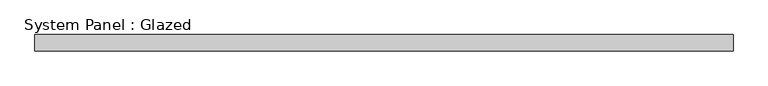
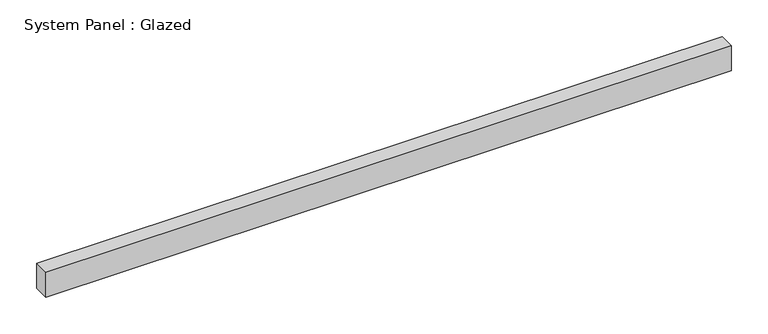
"""IFC4 building model written with IfcOpenShell, lengths in millimetres: plate geometry, System Panel : Glazed."""

import ifcopenshell
import ifcopenshell.guid

model = None  # the IFC model being written
_history = None  # IfcOwnerHistory: only IFC2X3 demands one
_inside = {}  # id of a spatial element -> (the spatial element, [elements in it])
_under = {}  # id of a project, library or spatial element -> (it, [spatial elements below it])
_declared = {}  # id of a project -> (the project, [libraries it declares])
_typed = {}  # id of a type object -> (the type object, [elements of that type])
_made_of = {}  # id of a material, layer set ... -> (it, [elements and type objects made of it])


def new_model(schema):
    """Start an empty IFC model of exactly this schema.

    Asked for "IFC4X3", IfcOpenShell would pick the latest addendum, in which some entities
    have other attributes; the version numbers below select the first issue.
    IFC2X3 requires an IfcOwnerHistory on every rooted entity: one is made here for all.
    """
    global model, _history
    if schema == "IFC4X3":
        model = ifcopenshell.file(schema_version=(4, 3, 0, 0))
    else:
        model = ifcopenshell.file(schema=schema)
    _inside.clear()
    _under.clear()
    _declared.clear()
    _typed.clear()
    _made_of.clear()
    _history = None
    if model.schema == "IFC2X3":
        org = make("IfcOrganization", Name="unknown")
        user = make(
            "IfcPersonAndOrganization",
            ThePerson=make("IfcPerson", FamilyName="unknown"),
            TheOrganization=org,
        )
        app = make(
            "IfcApplication",
            ApplicationDeveloper=org,
            Version="unknown",
            ApplicationFullName="unknown",
            ApplicationIdentifier="unknown",
        )
        _history = make(
            "IfcOwnerHistory",
            OwningUser=user,
            OwningApplication=app,
            ChangeAction="ADDED",
            CreationDate=0,
        )
    return model


def make(cls, **values):
    """One entity of the class cls with the attributes given. An attribute that is None is left unset."""
    return model.create_entity(
        cls, **{name: value for name, value in values.items() if value is not None}
    )


def rooted(cls, **values):
    """An entity with a GlobalId (a new one), such as an element, a storey or a relation."""
    return make(cls, GlobalId=ifcopenshell.guid.new(), OwnerHistory=_history, **values)


def si_unit(unit_type, name, prefix=None):
    """IfcSIUnit, for example si_unit("LENGTHUNIT", "METRE", prefix="MILLI")."""
    return make("IfcSIUnit", UnitType=unit_type, Prefix=prefix, Name=name)


def assignment(units):
    """IfcUnitAssignment: the units of a project."""
    return None if units is None else make("IfcUnitAssignment", Units=units)


def point(xyz):
    """IfcCartesianPoint."""
    return None if xyz is None else make("IfcCartesianPoint", Coordinates=xyz)


def direction(xyz):
    """IfcDirection."""
    return None if xyz is None else make("IfcDirection", DirectionRatios=xyz)


def frame(location, z_axis=None, x_axis=None):
    """IfcAxis2Placement3D, a coordinate frame: its origin and axes. An axis left out is left unset."""
    return make(
        "IfcAxis2Placement3D",
        Location=point(location),
        Axis=direction(z_axis),
        RefDirection=direction(x_axis),
    )


def origin():
    """The frame at (0, 0, 0) with its axes left unset."""
    return frame((0.0, 0.0, 0.0))


def origin_with_axes():
    """The frame at (0, 0, 0) with the z axis (0, 0, 1) and the x axis (1, 0, 0) written out."""
    return frame((0.0, 0.0, 0.0), z_axis=(0.0, 0.0, 1.0), x_axis=(1.0, 0.0, 0.0))


def place(relative_to, where):
    """IfcLocalPlacement: puts the frame where relative to a parent placement (None: the world)."""
    return make(
        "IfcLocalPlacement", PlacementRelTo=relative_to, RelativePlacement=where
    )


def context(
    kind, dimensions, precision=None, world=None, true_north=None, identifier=None
):
    """IfcGeometricRepresentationContext, for example the 3D "Model" context."""
    return make(
        "IfcGeometricRepresentationContext",
        ContextIdentifier=identifier,
        ContextType=kind,
        CoordinateSpaceDimension=dimensions,
        Precision=precision,
        WorldCoordinateSystem=world,
        TrueNorth=true_north,
    )


def project(units=None, contexts=None):
    """IfcProject with its units and contexts."""
    return rooted(
        "IfcProject",
        Name="project",
        RepresentationContexts=contexts,
        UnitsInContext=assignment(units),
    )


def spatial(cls, under=None, at=None, **own):
    """A site, building, storey or space (cls), placed at a placement, below another one or the project."""
    s = rooted(cls, ObjectPlacement=at, **own)
    if under is not None:
        _under.setdefault(under.id(), (under, []))[1].append(s)
    return s


def polyline(points):
    """IfcPolyline through the points."""
    return make("IfcPolyline", Points=[point(p) for p in points])


def outline(outer, holes=None, kind="AREA"):
    """IfcArbitraryClosedProfileDef: a profile drawn as a closed curve; with holes, ...WithVoids."""
    if holes is None:
        return make("IfcArbitraryClosedProfileDef", ProfileType=kind, OuterCurve=outer)
    return make(
        "IfcArbitraryProfileDefWithVoids",
        ProfileType=kind,
        OuterCurve=outer,
        InnerCurves=holes,
    )


def extrude(swept, where, along, depth):
    """IfcExtrudedAreaSolid: the profile swept, set in the frame where, extruded along a direction by depth."""
    return make(
        "IfcExtrudedAreaSolid",
        SweptArea=swept,
        Position=where,
        ExtrudedDirection=direction(along),
        Depth=depth,
    )


def shape(context_of_items, identifier, shape_type, items):
    """IfcShapeRepresentation: the items that make up one representation, for example the "Body"."""
    return make(
        "IfcShapeRepresentation",
        ContextOfItems=context_of_items,
        RepresentationIdentifier=identifier,
        RepresentationType=shape_type,
        Items=items,
    )


def source(mapping_origin, context_of_items, identifier, shape_type, items):
    """IfcRepresentationMap: a shape defined once, which mapped items show again and again."""
    return make(
        "IfcRepresentationMap",
        MappingOrigin=mapping_origin,
        MappedRepresentation=shape(context_of_items, identifier, shape_type, items),
    )


def transform(
    local_origin,
    x_axis=None,
    y_axis=None,
    z_axis=None,
    scale=None,
    scale2=None,
    scale3=None,
    uniform=True,
):
    """IfcCartesianTransformationOperator3D, or its non-uniform kind. x_axis, y_axis, z_axis: its Axis1, 2, 3."""
    if uniform:
        return make(
            "IfcCartesianTransformationOperator3D",
            Axis1=direction(x_axis),
            Axis2=direction(y_axis),
            LocalOrigin=point(local_origin),
            Scale=scale,
            Axis3=direction(z_axis),
        )
    return make(
        "IfcCartesianTransformationOperator3DnonUniform",
        Axis1=direction(x_axis),
        Axis2=direction(y_axis),
        LocalOrigin=point(local_origin),
        Scale=scale,
        Axis3=direction(z_axis),
        Scale2=scale2,
        Scale3=scale3,
    )


def mapped(mapping_source, mapping_target):
    """IfcMappedItem: shows the shape of a source again, moved by a transform."""
    return make(
        "IfcMappedItem", MappingSource=mapping_source, MappingTarget=mapping_target
    )


def made_of(thing, what):
    """Note that an element or type object is made of a material, layer set ...; save() writes the relation."""
    if what is not None:
        _made_of.setdefault(what.id(), (what, []))[1].append(thing)
    return thing


def element(
    cls,
    number,
    at=None,
    inside=None,
    cuts=None,
    type_object=None,
    material=None,
    context=None,
    identifier="Body",
    shape_type=None,
    held_by="IfcProductDefinitionShape",
    body=None,
    shapes=None,
    **own,
):
    """One element of the class cls, such as IfcWall. Its Tag is "e" and its number.

    at: its placement. inside: the storey or other place that contains it. cuts: it is an
    opening in that element (IfcRelVoidsElement). A single representation is given by context,
    identifier, shape_type and body (its items); several are given by shapes. held_by: the class
    of the entity that holds the representations. save() writes the other relations.
    """
    e = rooted(cls, Tag="e%d" % number, ObjectPlacement=at, **own)
    if body is not None:
        shapes = [shape(context, identifier, shape_type, body)]
    if shapes is not None:
        e.Representation = make(held_by, Representations=shapes)
    if inside is not None:
        _inside.setdefault(inside.id(), (inside, []))[1].append(e)
    if cuts is not None:
        rooted(
            "IfcRelVoidsElement", RelatingBuildingElement=cuts, RelatedOpeningElement=e
        )
    if type_object is not None:
        _typed.setdefault(type_object.id(), (type_object, []))[1].append(e)
    return made_of(e, material)


def aggregate(whole, parts):
    """IfcRelAggregates: a whole, such as a stair, and the parts it consists of."""
    return rooted("IfcRelAggregates", RelatingObject=whole, RelatedObjects=parts)


def save(model, path):
    """Write the relations noted so far, then the file.

    IfcRelAggregates (storeys below a building ...), IfcRelContainedInSpatialStructure (elements
    in a storey), IfcRelDefinesByType, IfcRelAssociatesMaterial and IfcRelDeclares: one each for
    every whole, place, type object, material and project.
    """
    for whole, parts in _under.values():
        aggregate(whole, parts)
    for where, things in _inside.values():
        rooted(
            "IfcRelContainedInSpatialStructure",
            RelatedElements=things,
            RelatingStructure=where,
        )
    for kind, things in _typed.values():
        rooted("IfcRelDefinesByType", RelatedObjects=things, RelatingType=kind)
    for what, things in _made_of.values():
        rooted("IfcRelAssociatesMaterial", RelatedObjects=things, RelatingMaterial=what)
    for by, libraries in _declared.values():
        rooted("IfcRelDeclares", RelatingContext=by, RelatedDefinitions=libraries)
    model.write(path)


def system_panel_glazed_5c475300(model_context):
    return source(origin(), model_context, "Body", "SweptSolid", [
        extrude(outline(polyline([(542.0483058, -44.45), (-542.0483058, -44.45), (-542.0483058, -19.05), (542.0483058, -19.05), (542.0483058, -44.45)])), origin_with_axes(), (0.0, 0.0, 1.0), 41.9143134),
    ])


if __name__ == "__main__":
    model = new_model("IFC4")
    model_context = context("Model", 3, world=origin())
    ifc_project = project(units=[si_unit("LENGTHUNIT", "METRE", prefix="MILLI")], contexts=[model_context])
    site = spatial("IfcSite", under=ifc_project)
    building = spatial("IfcBuilding", under=site)
    placement = place(None, origin())
    system_panel_glazed_shape = system_panel_glazed_5c475300(model_context)
    element("IfcPlate", 1, ObjectType="System Panel : Glazed", at=placement, inside=building, context=model_context, shape_type="MappedRepresentation", body=[
        mapped(system_panel_glazed_shape, transform((0.0, 0.0, 0.0), x_axis=(1.0, 0.0, 0.0), y_axis=(0.0, 1.0, 0.0), z_axis=(0.0, 0.0, 1.0))),
    ])
    save(model, "model.ifc")

# Revit data of these elements
# Type "System Panel : Glazed"
#   Construction Type Id = "GSP4R"
#   Analytic Construction = "1/8 in Pilkington single glazing"
#   Visual Light Transmittance = 0.9
#   Solar Heat Gain Coefficient = 0.86
#   Heat Transfer Coefficient (U) = 1.18115 BTU/(h·ft²·°F)
#   Define Thermal Properties by = 1
# Element 1 (IfcPlate, "System Panel : Glazed")
#   Materials on its faces: "Glass"
# Materials
#   "Glass": class "Glass", colour RGB 0 128 192, transparency 0.75, Description = "Soda Lime Glass", Cost = 0
